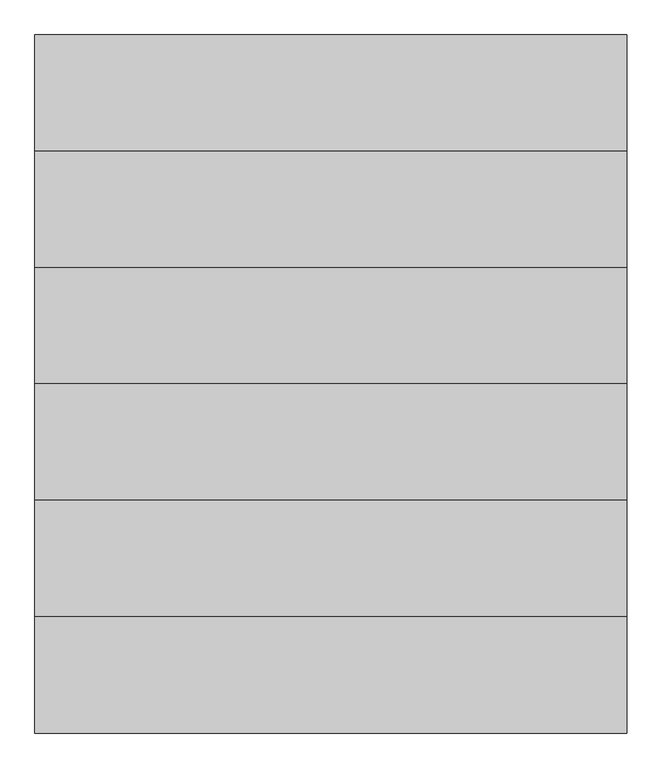
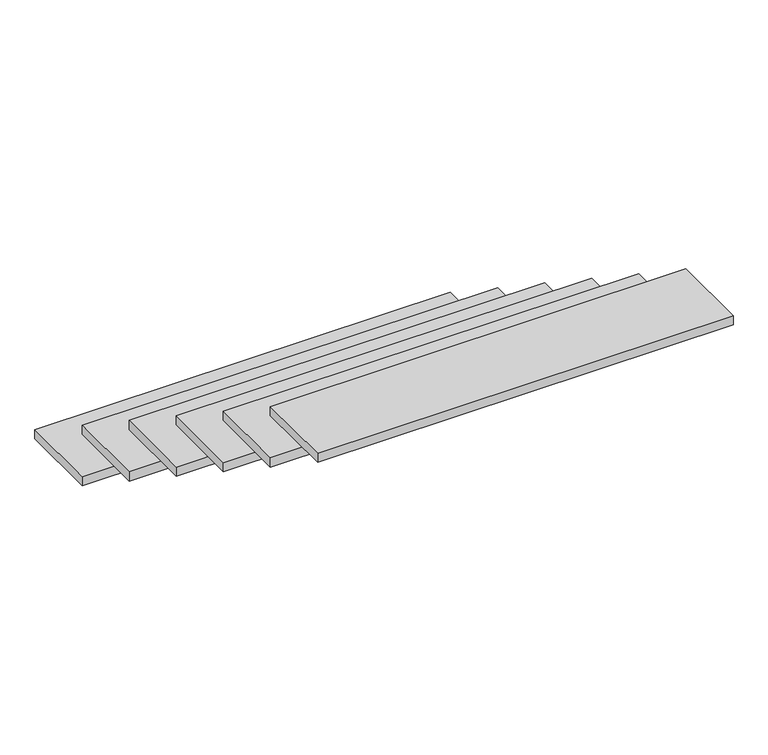
"""IFC4 building model written with IfcOpenShell, lengths in millimetres: stair flight geometry."""

from ifc_helpers import new_model, si_unit, frame, origin, place, context, project, spatial, polyline, outline, extrude, source, transform, mapped, element, save


def stair_flight_b88c65ee(model_context):
    return source(origin(), model_context, "Body", "SweptSolid", [
        extrude(outline(polyline([(13552.1845799, 2149.5208589), (12177.1845799, 2149.5208589), (12177.1845799, 2419.5208589), (13552.1845799, 2419.5208589), (13552.1845799, 2149.5208589)])), frame((0.0, 0.0, 7967.9618634), z_axis=(0.0, 0.0, 1.0), x_axis=(1.0, 0.0, 0.0)), (0.0, 0.0, 1.0), 32.0),
        extrude(outline(polyline([(13552.1845799, 1879.5208589), (12177.1845799, 1879.5208589), (12177.1845799, 2149.5208589), (13552.1845799, 2149.5208589), (13552.1845799, 1879.5208589)])), frame((0.0, 0.0, 8147.9618634), z_axis=(0.0, 0.0, 1.0), x_axis=(1.0, 0.0, 0.0)), (0.0, 0.0, 1.0), 32.0),
        extrude(outline(polyline([(13552.1845799, 1609.5208589), (12177.1845799, 1609.5208589), (12177.1845799, 1879.5208589), (13552.1845799, 1879.5208589), (13552.1845799, 1609.5208589)])), frame((0.0, 0.0, 8327.9618634), z_axis=(0.0, 0.0, 1.0), x_axis=(1.0, 0.0, 0.0)), (0.0, 0.0, 1.0), 32.0),
        extrude(outline(polyline([(13552.1845799, 1339.5208589), (12177.1845799, 1339.5208589), (12177.1845799, 1609.5208589), (13552.1845799, 1609.5208589), (13552.1845799, 1339.5208589)])), frame((0.0, 0.0, 8507.9618634), z_axis=(0.0, 0.0, 1.0), x_axis=(1.0, 0.0, 0.0)), (0.0, 0.0, 1.0), 32.0),
        extrude(outline(polyline([(13552.1845799, 1069.5208589), (12177.1845799, 1069.5208589), (12177.1845799, 1339.5208589), (13552.1845799, 1339.5208589), (13552.1845799, 1069.5208589)])), frame((0.0, 0.0, 8687.9618634), z_axis=(0.0, 0.0, 1.0), x_axis=(1.0, 0.0, 0.0)), (0.0, 0.0, 1.0), 32.0),
        extrude(outline(polyline([(13552.1845799, 799.5208589), (12177.1845799, 799.5208589), (12177.1845799, 1069.5208589), (13552.1845799, 1069.5208589), (13552.1845799, 799.5208589)])), frame((0.0, 0.0, 8867.9618634), z_axis=(0.0, 0.0, 1.0), x_axis=(1.0, 0.0, 0.0)), (0.0, 0.0, 1.0), 32.0),
    ])


if __name__ == "__main__":
    model = new_model("IFC4")
    model_context = context("Model", 3, world=origin())
    ifc_project = project(units=[si_unit("LENGTHUNIT", "METRE", prefix="MILLI")], contexts=[model_context])
    site = spatial("IfcSite", under=ifc_project)
    building = spatial("IfcBuilding", under=site)
    placement = place(None, origin())
    stair_flight_shape = stair_flight_b88c65ee(model_context)
    element("IfcStairFlight", 1, at=placement, inside=building, context=model_context, shape_type="MappedRepresentation", body=[
        mapped(stair_flight_shape, transform((0.0, 0.0, 0.0), x_axis=(1.0, 0.0, 0.0), y_axis=(0.0, 1.0, 0.0), z_axis=(0.0, 0.0, 1.0))),
    ])
    save(model, "model.ifc")
